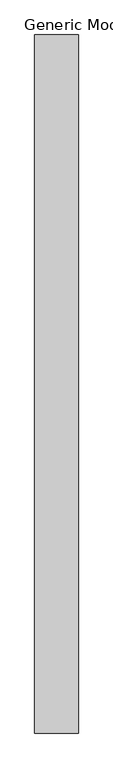
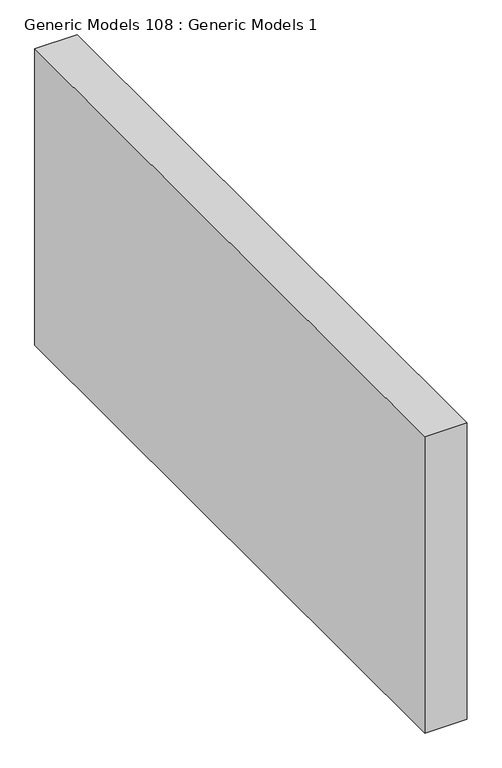
"""IFC4 building model written with IfcOpenShell, lengths in millimetres: proxy geometry, Generic Models 108 : Generic Models 1."""

from ifc_helpers import new_model, si_unit, frame, origin, place, context, project, spatial, polyline, outline, extrude, source, transform, mapped, element, save


def generic_models_108_generic_models_1_496acf5e(model_context):
    return source(origin(), model_context, "Body", "SweptSolid", [
        extrude(outline(polyline([(52216.05, 1219.2), (52216.05, 0.0), (52139.85, 0.0), (52139.85, 1219.2), (52216.05, 1219.2)])), frame((0.0, 0.0, 4570.4125), z_axis=(0.0, 0.0, 1.0), x_axis=(1.0, 0.0, 0.0)), (0.0, 0.0, 1.0), 565.15),
    ])


if __name__ == "__main__":
    model = new_model("IFC4")
    model_context = context("Model", 3, world=origin())
    ifc_project = project(units=[si_unit("LENGTHUNIT", "METRE", prefix="MILLI")], contexts=[model_context])
    site = spatial("IfcSite", under=ifc_project)
    building = spatial("IfcBuilding", under=site)
    placement = place(None, origin())
    generic_models_108_generic_models_1_shape = generic_models_108_generic_models_1_496acf5e(model_context)
    element("IfcBuildingElementProxy", 1, Name="Generic Models 108 : Generic Models 1", ObjectType="Generic Models 108 : Generic Models 1", at=placement, inside=building, context=model_context, shape_type="MappedRepresentation", body=[
        mapped(generic_models_108_generic_models_1_shape, transform((0.0, 0.0, 0.0), x_axis=(1.0, 0.0, 0.0), y_axis=(0.0, 1.0, 0.0), z_axis=(0.0, 0.0, 1.0))),
    ])
    save(model, "model.ifc")

# Revit data of these elements
# Element 1 (IfcBuildingElementProxy, "Generic Models 108 : Generic Models 1")
#   Materials on its faces: "(S) SOUND BATT. INSULATION (THICKNESS TO MATCH WALL DEPTH)"
# Materials
#   "(S) SOUND BATT. INSULATION (THICKNESS TO MATCH WALL DEPTH)": class "Unassigned", colour RGB 255 255 255, transparency 0, Cost = 0
